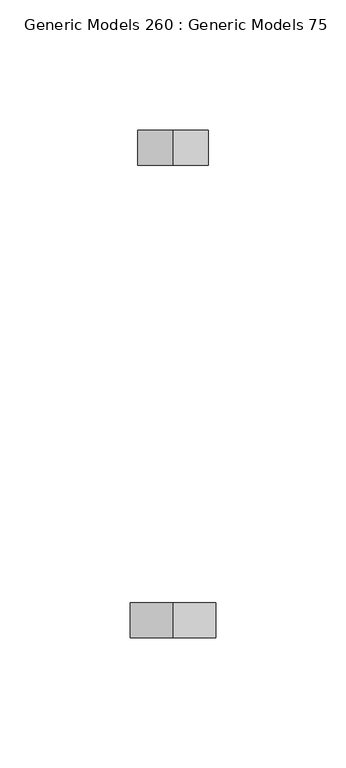
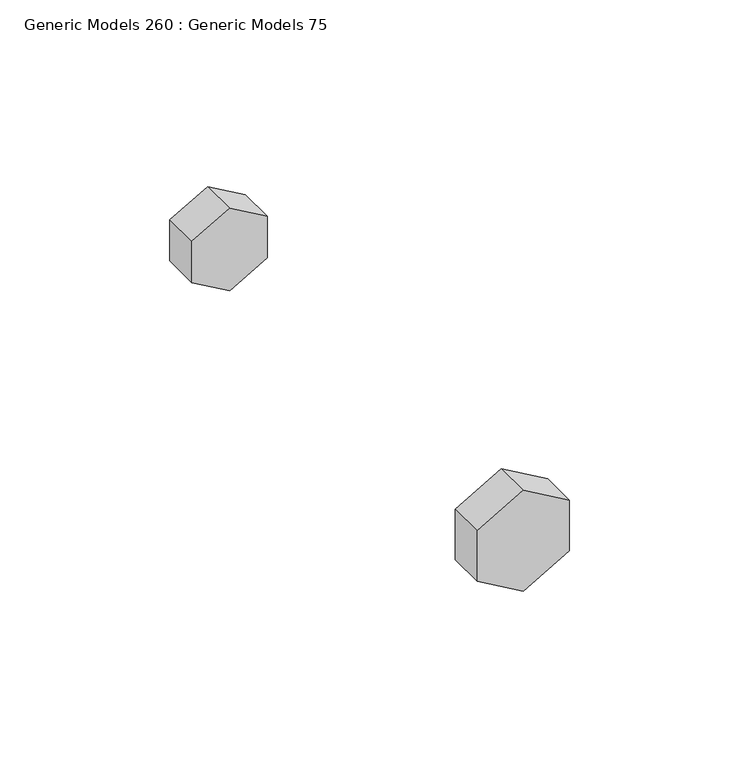
"""IFC4 building model written with IfcOpenShell, lengths in millimetres: proxy geometry, Generic Models 260 : Generic Models 75."""

from ifc_helpers import new_model, si_unit, frame, origin, place, context, project, spatial, polyline, outline, extrude, source, transform, mapped, element, save


def generic_models_260_generic_models_75_7a27c1cf(model_context):
    return source(origin(), model_context, "Body", "SweptSolid", [
        extrude(outline(polyline([(266616.830998, 32006.2068618), (266635.880998, 32006.2068618), (266645.405998, 31989.7090778), (266635.880998, 31973.2112939), (266616.830998, 31973.2112939), (266607.305998, 31989.7090778), (266616.830998, 32006.2068618)])), frame((0.0, 30676.7094112, 0.0), z_axis=(0.0, 1.0, 0.0), x_axis=(0.0, 0.0, 1.0)), (0.0, 0.0, 1.0), 13.49375),
        extrude(outline(polyline([(266633.9638403, 31976.2187024), (266618.3864965, 31976.2187024), (266610.5978246, 31989.7090778), (266618.3864965, 32003.1994532), (266633.9638403, 32003.1994532), (266641.7525121, 31989.7090778), (266633.9638403, 31976.2187024)])), frame((0.0, 30858.4781612, 0.0), z_axis=(0.0, 1.0, 0.0), x_axis=(0.0, 0.0, 1.0)), (0.0, 0.0, 1.0), 13.49375),
    ])


if __name__ == "__main__":
    model = new_model("IFC4")
    model_context = context("Model", 3, world=origin())
    ifc_project = project(units=[si_unit("LENGTHUNIT", "METRE", prefix="MILLI")], contexts=[model_context])
    site = spatial("IfcSite", under=ifc_project)
    building = spatial("IfcBuilding", under=site)
    placement = place(None, origin())
    generic_models_260_generic_models_75_shape = generic_models_260_generic_models_75_7a27c1cf(model_context)
    element("IfcBuildingElementProxy", 1, Name="Generic Models 260 : Generic Models 75", ObjectType="Generic Models 260 : Generic Models 75", at=placement, inside=building, context=model_context, shape_type="MappedRepresentation", body=[
        mapped(generic_models_260_generic_models_75_shape, transform((0.0, 0.0, 0.0), x_axis=(1.0, 0.0, 0.0), y_axis=(0.0, 1.0, 0.0), z_axis=(0.0, 0.0, 1.0))),
    ])
    save(model, "model.ifc")

# Revit data of these elements
# Element 1 (IfcBuildingElementProxy, "Generic Models 260 : Generic Models 75")
#   Materials on its faces: "3/4\" GALV. THRU BOLTS"
# Materials
#   "3/4\" GALV. THRU BOLTS": class "Generic", colour RGB 105 69 171, transparency 0, Cost = 0
